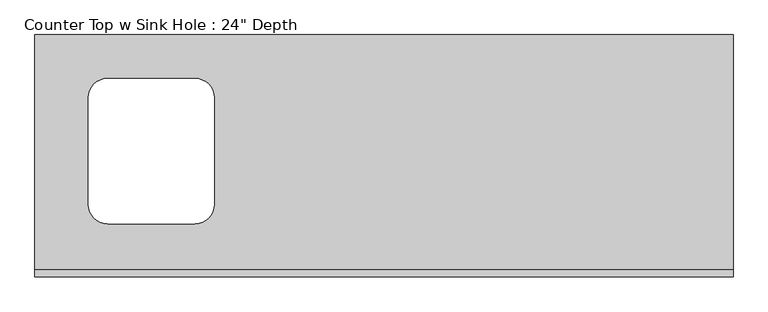
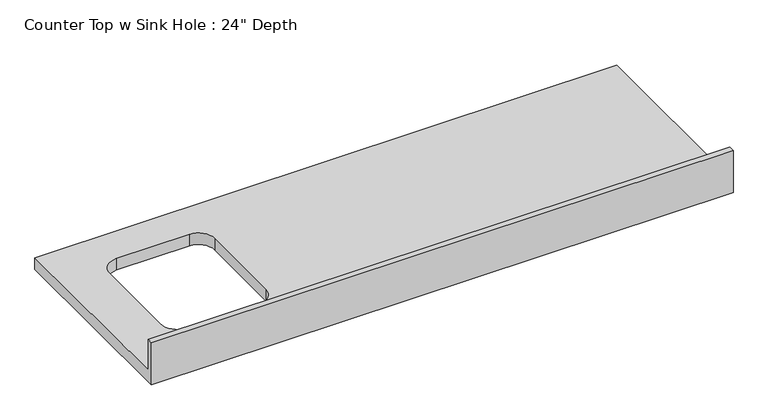
"""IFC4 building model written with IfcOpenShell, lengths in millimetres: furniture geometry."""

from ifc_helpers import new_model, si_unit, frame, origin, place, context, project, spatial, polyline, circle_curve, source, transform, mapped, element, save
from ifc_brep_helpers import plane_surface, revolved_surface, advanced_brep


def furniture_1408e768(model_context):
    return source(origin(), model_context, "Body", "AdvancedBrep", [
        advanced_brep(
        [(-1200.4622951, 635.0, 914.4), (-1200.4622951, 19.05, 914.4), (628.3377049, 19.05, 914.4), (628.3377049, 635.0, 914.4), (-1009.9622951, 139.7, 914.4), (-1060.7622951, 190.5, 914.4), (-1060.7622951, 469.9, 914.4), (-1009.9622951, 520.7, 914.4), (-781.3622951, 520.7, 914.4), (-730.5622951, 469.9, 914.4), (-730.5622951, 190.5, 914.4), (-781.3622951, 139.7, 914.4), (628.3377049, 0.0, 876.3), (-1200.4622951, 0.0, 876.3), (-1200.4622951, 635.0, 876.3), (628.3377049, 635.0, 876.3), (-781.3622951, 139.7, 876.3), (-730.5622951, 190.5, 876.3), (-730.5622951, 469.9, 876.3), (-781.3622951, 520.7, 876.3), (-1009.9622951, 520.7, 876.3), (-1060.7622951, 469.9, 876.3), (-1060.7622951, 190.5, 876.3), (-1009.9622951, 139.7, 876.3), (628.3377049, 0.0, 1016.0), (-1200.4622951, 0.0, 1016.0), (-1200.4622951, 19.05, 1016.0), (628.3377049, 19.05, 1016.0)],
        [
            (0, 1),
            (1, 2),
            (2, 3),
            (3, 0),
            (4, 5, circle_curve(frame((-1009.9622951, 190.5, 914.4), z_axis=(0.0, 0.0, -1.0), x_axis=(1.0, 0.0, 0.0)), 50.8)),
            (5, 6),
            (6, 7, circle_curve(frame((-1009.9622951, 469.9, 914.4), z_axis=(0.0, 0.0, -1.0), x_axis=(1.0, 0.0, 0.0)), 50.8)),
            (7, 8),
            (8, 9, circle_curve(frame((-781.3622951, 469.9, 914.4), z_axis=(0.0, 0.0, -1.0), x_axis=(1.0, 0.0, 0.0)), 50.8)),
            (9, 10),
            (10, 11, circle_curve(frame((-781.3622951, 190.5, 914.4), z_axis=(0.0, 0.0, -1.0), x_axis=(1.0, 0.0, 0.0)), 50.8)),
            (11, 4),
            (12, 13),
            (13, 14),
            (14, 15),
            (15, 12),
            (16, 17, circle_curve(frame((-781.3622951, 190.5, 876.3), z_axis=(0.0, 0.0, 1.0), x_axis=(1.0, 0.0, 0.0)), 50.8)),
            (17, 18),
            (18, 19, circle_curve(frame((-781.3622951, 469.9, 876.3), z_axis=(0.0, 0.0, 1.0), x_axis=(1.0, 0.0, 0.0)), 50.8)),
            (19, 20),
            (20, 21, circle_curve(frame((-1009.9622951, 469.9, 876.3), z_axis=(0.0, 0.0, 1.0), x_axis=(1.0, 0.0, 0.0)), 50.8)),
            (21, 22),
            (22, 23, circle_curve(frame((-1009.9622951, 190.5, 876.3), z_axis=(0.0, 0.0, 1.0), x_axis=(1.0, 0.0, 0.0)), 50.8)),
            (23, 16),
            (12, 24),
            (24, 25),
            (25, 13),
            (25, 26),
            (26, 1),
            (0, 14),
            (3, 15),
            (2, 27),
            (27, 24),
            (11, 16),
            (23, 4),
            (22, 5),
            (21, 6),
            (20, 7),
            (19, 8),
            (18, 9),
            (17, 10),
            (27, 26),
        ],
        [
            plane_surface(frame((-1200.4622951, 0.0, 914.4), z_axis=(0.0, 0.0, 1.0), x_axis=(-1.0, 0.0, 0.0))),
            plane_surface(frame((-1200.4622951, 0.0, 876.3), z_axis=(0.0, 0.0, -1.0), x_axis=(1.0, 0.0, 0.0))),
            plane_surface(frame((628.3377049, 0.0, 914.4), z_axis=(0.0, -1.0, 0.0), x_axis=(0.0, 0.0, -1.0))),
            plane_surface(frame((-1200.4622951, 0.0, 914.4), z_axis=(-1.0, 0.0, 0.0), x_axis=(0.0, 0.0, -1.0))),
            plane_surface(frame((-1200.4622951, 635.0, 914.4), z_axis=(0.0, 1.0, 0.0), x_axis=(0.0, 0.0, -1.0))),
            plane_surface(frame((628.3377049, 635.0, 914.4), z_axis=(1.0, 0.0, 0.0), x_axis=(0.0, 0.0, -1.0))),
            plane_surface(frame((-781.3622951, 139.7, 914.4), z_axis=(0.0, 1.0, 0.0), x_axis=(0.0, 0.0, -1.0))),
            revolved_surface(polyline([(-959.1622951, 190.5, 914.4), (-959.1622951, 190.5, 876.3)]), (-1009.9622951, 190.5, 876.3), (0.0, 0.0, 1.0)),
            plane_surface(frame((-1060.7622951, 190.5, 914.4), z_axis=(1.0, 0.0, 0.0), x_axis=(0.0, 0.0, -1.0))),
            revolved_surface(polyline([(-959.1622951, 469.9, 914.4), (-959.1622951, 469.9, 876.3)]), (-1009.9622951, 469.9, 876.3), (0.0, 0.0, 1.0)),
            plane_surface(frame((-1009.9622951, 520.7, 914.4), z_axis=(0.0, -1.0, 0.0), x_axis=(0.0, 0.0, -1.0))),
            revolved_surface(polyline([(-730.5622951, 469.9, 914.4), (-730.5622951, 469.9, 876.3)]), (-781.3622951, 469.9, 876.3), (0.0, 0.0, 1.0)),
            plane_surface(frame((-730.5622951, 469.9, 914.4), z_axis=(-1.0, 0.0, 0.0), x_axis=(0.0, 0.0, -1.0))),
            revolved_surface(polyline([(-730.5622951, 190.5, 914.4), (-730.5622951, 190.5, 876.3)]), (-781.3622951, 190.5, 876.3), (0.0, 0.0, 1.0)),
            plane_surface(frame((-1200.4622951, 0.0, 1016.0), z_axis=(0.0, 0.0, 1.0), x_axis=(0.0, 1.0, 0.0))),
            plane_surface(frame((-1200.4622951, 19.05, 1016.0), z_axis=(0.0, 1.0, 0.0), x_axis=(0.0, 0.0, -1.0))),
        ],
        [
            (0, [[1, 2, 3, 4], [5, 6, 7, 8, 9, 10, 11, 12]]),
            (1, [[13, 14, 15, 16], [17, 18, 19, 20, 21, 22, 23, 24]]),
            (2, [[25, 26, 27, -13]]),
            (3, [[-27, 28, 29, -1, 30, -14]]),
            (4, [[31, -15, -30, -4]]),
            (5, [[-31, -3, 32, 33, -25, -16]]),
            (6, [[-12, 34, -24, 35]]),
            (7, [[-23, 36, -5, -35]]),
            (8, [[-22, 37, -6, -36]]),
            (9, [[-21, 38, -7, -37]]),
            (10, [[-20, 39, -8, -38]]),
            (11, [[-19, 40, -9, -39]]),
            (12, [[-18, 41, -10, -40]]),
            (13, [[-11, -41, -17, -34]]),
            (14, [[-26, -33, 42, -28]]),
            (15, [[-32, -2, -29, -42]]),
        ],
    ),
    ])


if __name__ == "__main__":
    model = new_model("IFC4")
    model_context = context("Model", 3, world=origin())
    ifc_project = project(units=[si_unit("LENGTHUNIT", "METRE", prefix="MILLI")], contexts=[model_context])
    site = spatial("IfcSite", under=ifc_project)
    building = spatial("IfcBuilding", under=site)
    placement = place(None, origin())
    furniture_shape = furniture_1408e768(model_context)
    element("IfcFurniture", 1, ObjectType="Counter Top w Sink Hole : 24\" Depth", at=placement, inside=building, context=model_context, shape_type="MappedRepresentation", body=[
        mapped(furniture_shape, transform((0.0, 0.0, 0.0), x_axis=(1.0, 0.0, 0.0), y_axis=(0.0, 1.0, 0.0), z_axis=(0.0, 0.0, 1.0))),
    ])
    save(model, "model.ifc")

# Revit data of these elements
# Type "Counter Top w Sink Hole : 24\" Depth"
#   Assembly Code = "C1030400"
#   Counter Thickness = 0' - 1 1/2"
#   Depth = 2' - 1"
#   Height = 3' - 0"
#   Length [instance default] = 8' - 0"
#   Sink Location [instance default] = 2' - 0"
#   Sink Location To Wall [instance default] = 0' - 6"
#   Sink Opening Depth [instance default] = 1' - 3"
#   Sink Opening Width [instance default] = 2' - 3"
#   Counter Top Material = none
#   Default Elevation = 0
# Element 1 (IfcFurniture, "Counter Top w Sink Hole : 24\" Depth")
#   Length = 6' - 0"
#   Sink Location = 1' - 0"
#   Sink Opening Depth = 1' - 2"
#   Sink Opening Width = 1' - 0"
#   Materials on its faces: "Counter Top"
# Materials
#   "Counter Top": class "Unassigned", colour RGB 226 177 128, transparency 0
